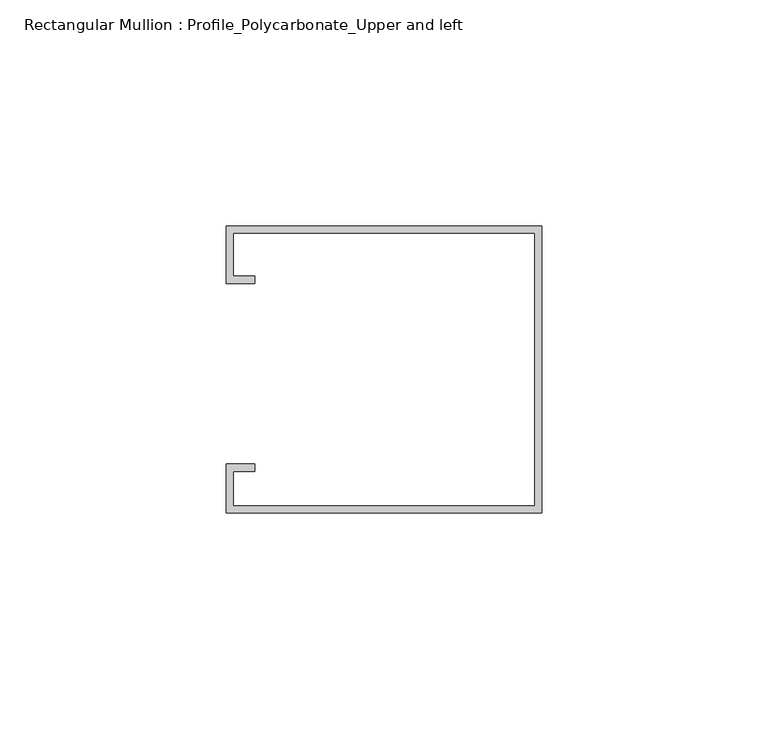
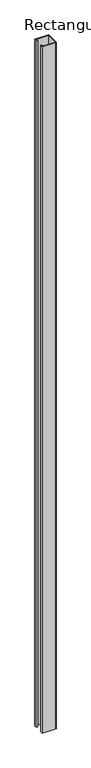
"""IFC4 building model written with IfcOpenShell, lengths in millimetres: member geometry, Rectangular Mullion : Profile_Polycarbonate_Upper and left."""

from ifc_helpers import new_model, si_unit, frame, origin, place, context, project, spatial, polyline, outline, extrude, source, transform, mapped, element, save


def rectangular_mullion_profile_polycarbonate_upper_and_left_ee42aaf8(model_context):
    return source(origin(), model_context, "Body", "SweptSolid", [
        extrude(outline(polyline([(0.0, 32.7), (0.0, -30.8), (-69.85, -30.8), (-69.85, -20.0), (-63.5, -20.0), (-63.5, -21.5875), (-68.2625, -21.5875), (-68.2625, -29.2125), (-1.5875, -29.2125), (-1.5875, 31.1125), (-68.2625, 31.1125), (-68.2625, 21.5875), (-63.5, 21.5875), (-63.5, 20.0), (-69.85, 20.0), (-69.85, 32.7), (0.0, 32.7)])), frame((0.0, 0.0, -3657.6), z_axis=(0.0, 0.0, 1.0), x_axis=(1.0, 0.0, 0.0)), (0.0, 0.0, 1.0), 3657.6),
    ])


if __name__ == "__main__":
    model = new_model("IFC4")
    model_context = context("Model", 3, world=origin())
    ifc_project = project(units=[si_unit("LENGTHUNIT", "METRE", prefix="MILLI")], contexts=[model_context])
    site = spatial("IfcSite", under=ifc_project)
    building = spatial("IfcBuilding", under=site)
    placement = place(None, origin())
    rectangular_mullion_profile_polycarbonate_upper_and_left_shape = rectangular_mullion_profile_polycarbonate_upper_and_left_ee42aaf8(model_context)
    element("IfcMember", 1, ObjectType="Rectangular Mullion : Profile_Polycarbonate_Upper and left", at=placement, inside=building, context=model_context, shape_type="MappedRepresentation", body=[
        mapped(rectangular_mullion_profile_polycarbonate_upper_and_left_shape, transform((0.0, 0.0, 0.0), x_axis=(1.0, 0.0, 0.0), y_axis=(0.0, 1.0, 0.0), z_axis=(0.0, 0.0, 1.0))),
    ])
    save(model, "model.ifc")

# Revit data of these elements
# Type "Rectangular Mullion : Profile_Polycarbonate_Upper and left"
#   built-in parameter 1007322 = 0.208333 (stored number, unit not read)
#   built-in parameter 1007321 = 0.00520833 (stored number, unit not read)
#   built-in parameter 1007320 = 0 (stored number, unit not read)
# Element 1 (IfcMember, "Rectangular Mullion : Profile_Polycarbonate_Upper and left")
#   Materials on its faces: "ALUMINUM PROFILE AT POLYCARBONATE PANEL"
# Materials
#   "ALUMINUM PROFILE AT POLYCARBONATE PANEL": class "Metal", colour RGB 244 244 244, transparency 0, Description = "Aluminum 6061", Cost = 0
